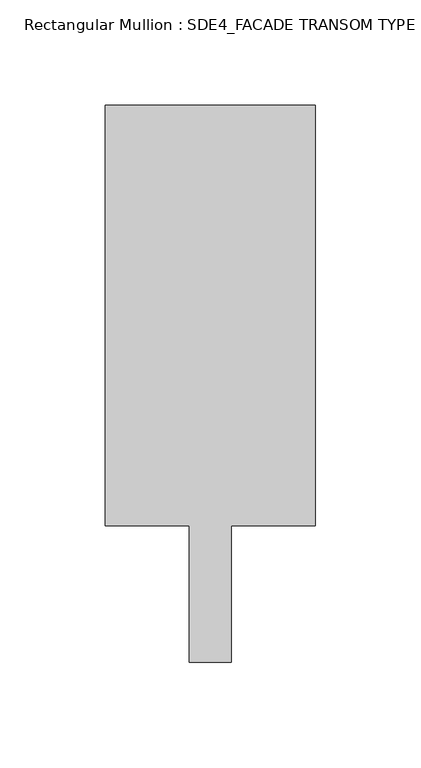
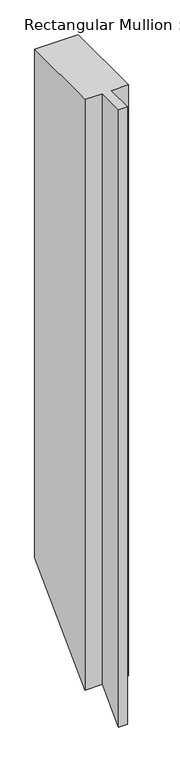
"""IFC4 building model written with IfcOpenShell, lengths in millimetres: member geometry, Rectangular Mullion : SDE4_FACADE TRANSOM TYPE 2."""

from ifc_helpers import new_model, si_unit, origin, place, context, project, spatial, faceted_brep, source, transform, mapped, element, save


def rectangular_mullion_sde4_facade_transom_type_2_dbd0d076(model_context):
    return source(origin(), model_context, "Body", "Brep", [
        faceted_brep([(50.0, 132.5, 0.0), (-50.0, 132.5, 0.0), (-50.0, -67.5, 0.0), (-10.0, -67.5, 0.0), (-10.0, -132.5, 0.0), (10.0, -132.5, 0.0), (10.0, -67.5, 0.0), (50.0, -67.5, 0.0), (50.0, 132.5, -1233.75), (-50.0, 132.5, -1233.75), (-50.0, -67.5, -1433.75), (-10.0, -67.5, -1433.75), (-10.0, -132.5, -1498.75), (10.0, -132.5, -1498.75), (10.0, -67.5, -1433.75), (50.0, -67.5, -1433.75)], [[[0, 1, 2, 3, 4, 5, 6, 7]], [[1, 0, 8, 9]], [[2, 1, 9, 10]], [[3, 2, 10, 11]], [[4, 3, 11, 12]], [[5, 4, 12, 13]], [[6, 5, 13, 14]], [[7, 6, 14, 15]], [[0, 7, 15, 8]], [[8, 15, 14, 13, 12, 11, 10, 9]]]),
    ])


if __name__ == "__main__":
    model = new_model("IFC4")
    model_context = context("Model", 3, world=origin())
    ifc_project = project(units=[si_unit("LENGTHUNIT", "METRE", prefix="MILLI")], contexts=[model_context])
    site = spatial("IfcSite", under=ifc_project)
    building = spatial("IfcBuilding", under=site)
    placement = place(None, origin())
    rectangular_mullion_sde4_facade_transom_type_2_shape = rectangular_mullion_sde4_facade_transom_type_2_dbd0d076(model_context)
    element("IfcMember", 1, ObjectType="Rectangular Mullion : SDE4_FACADE TRANSOM TYPE 2", at=placement, inside=building, context=model_context, shape_type="MappedRepresentation", body=[
        mapped(rectangular_mullion_sde4_facade_transom_type_2_shape, transform((0.0, 0.0, 0.0), x_axis=(1.0, 0.0, 0.0), y_axis=(0.0, 1.0, 0.0), z_axis=(0.0, 0.0, 1.0))),
    ])
    save(model, "model.ifc")

# Revit data of these elements
# Type "Rectangular Mullion : SDE4_FACADE TRANSOM TYPE 2"
#   built-in parameter 1007322 = 0.869423 (stored number, unit not read)
#   built-in parameter 1007321 = 0.164042 (stored number, unit not read)
#   built-in parameter 1007320 = 0.164042 (stored number, unit not read)
